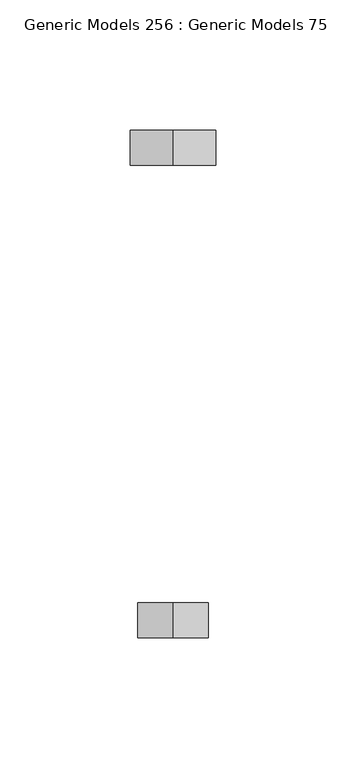
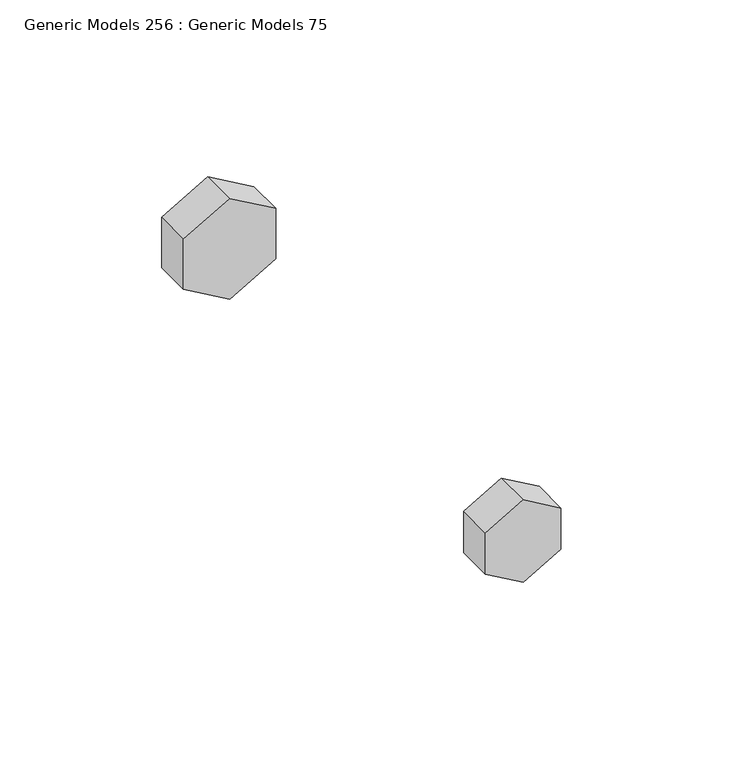
"""IFC4 building model written with IfcOpenShell, lengths in millimetres: proxy geometry, Generic Models 256 : Generic Models 75."""

from ifc_helpers import new_model, si_unit, frame, origin, place, context, project, spatial, polyline, outline, extrude, source, transform, mapped, element, save


def generic_models_256_generic_models_75_6f7e4d8f(model_context):
    return source(origin(), model_context, "Body", "SweptSolid", [
        extrude(outline(polyline([(266616.830998, 32006.2068618), (266635.880998, 32006.2068618), (266645.405998, 31989.7090778), (266635.880998, 31973.2112939), (266616.830998, 31973.2112939), (266607.305998, 31989.7090778), (266616.830998, 32006.2068618)])), frame((0.0, 35373.9582942, 0.0), z_axis=(0.0, 1.0, 0.0), x_axis=(0.0, 0.0, 1.0)), (0.0, 0.0, 1.0), 13.49375),
        extrude(outline(polyline([(266633.9638403, 31976.2187024), (266618.3864965, 31976.2187024), (266610.5978246, 31989.7090778), (266618.3864965, 32003.1994532), (266633.9638403, 32003.1994532), (266641.7525121, 31989.7090778), (266633.9638403, 31976.2187024)])), frame((0.0, 35192.1895442, 0.0), z_axis=(0.0, 1.0, 0.0), x_axis=(0.0, 0.0, 1.0)), (0.0, 0.0, 1.0), 13.49375),
    ])


if __name__ == "__main__":
    model = new_model("IFC4")
    model_context = context("Model", 3, world=origin())
    ifc_project = project(units=[si_unit("LENGTHUNIT", "METRE", prefix="MILLI")], contexts=[model_context])
    site = spatial("IfcSite", under=ifc_project)
    building = spatial("IfcBuilding", under=site)
    placement = place(None, origin())
    generic_models_256_generic_models_75_shape = generic_models_256_generic_models_75_6f7e4d8f(model_context)
    element("IfcBuildingElementProxy", 1, Name="Generic Models 256 : Generic Models 75", ObjectType="Generic Models 256 : Generic Models 75", at=placement, inside=building, context=model_context, shape_type="MappedRepresentation", body=[
        mapped(generic_models_256_generic_models_75_shape, transform((0.0, 0.0, 0.0), x_axis=(1.0, 0.0, 0.0), y_axis=(0.0, 1.0, 0.0), z_axis=(0.0, 0.0, 1.0))),
    ])
    save(model, "model.ifc")

# Revit data of these elements
# Element 1 (IfcBuildingElementProxy, "Generic Models 256 : Generic Models 75")
#   Materials on its faces: "3/4\" GALV. THRU BOLTS"
# Materials
#   "3/4\" GALV. THRU BOLTS": class "Generic", colour RGB 105 69 171, transparency 0, Cost = 0
